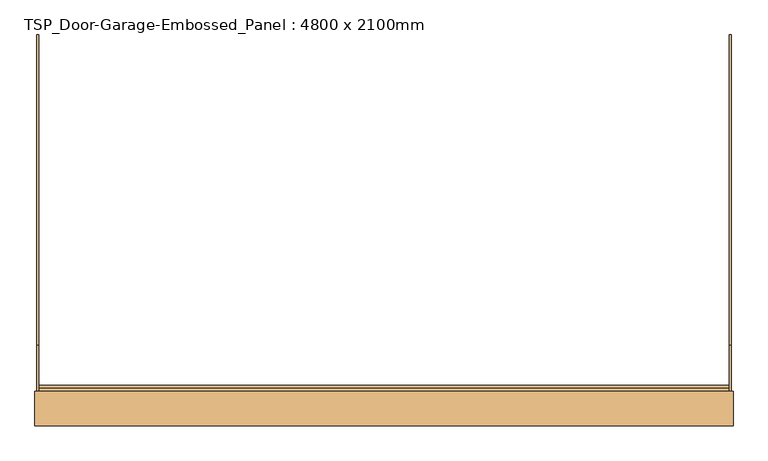
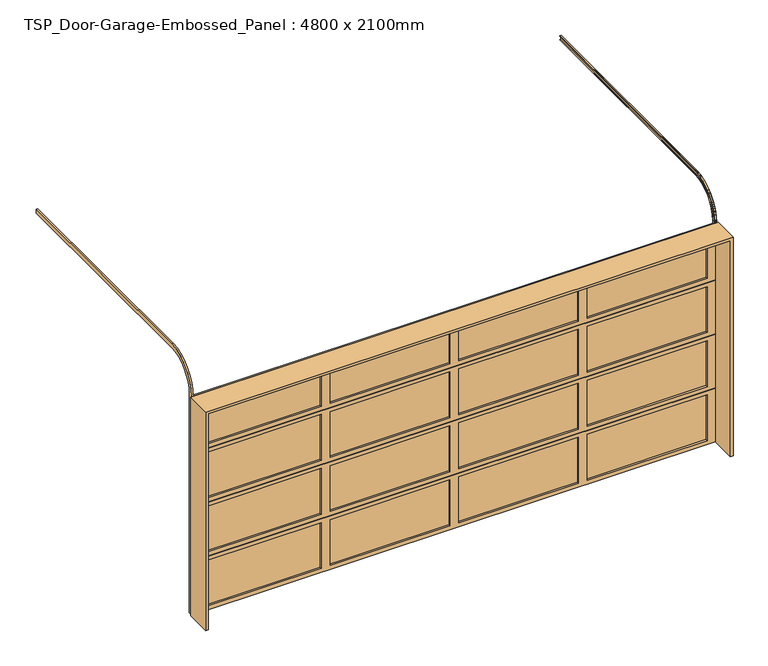
"""IFC4 building model written with IfcOpenShell, lengths in millimetres: door geometry, TSP_Door-Garage-Embossed_Panel : 4800 x 2100mm."""

from ifc_helpers import new_model, si_unit, frame, origin, place, context, project, spatial, polyline, circle_curve, outline, extrude, faceted_brep, source, transform, mapped, element, save
from ifc_brep_helpers import plane_surface, cylinder_surface, revolved_surface, advanced_brep


def tsp_door_garage_embossed_panel_4800_x_2100mm_f4924081(model_context):
    return source(origin(), model_context, "Body", "SolidModel", [
        extrude(outline(polyline([(1141.2666667, 140.0), (41.2666667, 140.0), (41.2666667, 146.35), (1141.2666667, 146.35), (1141.2666667, 140.0)])), frame((0.0, 0.0, 1615.0), z_axis=(0.0, 0.0, 1.0), x_axis=(1.0, 0.0, 0.0)), (0.0, 0.0, 1.0), 445.0),
        extrude(outline(polyline([(-41.2666667, 140.0), (-1141.2666667, 140.0), (-1141.2666667, 146.35), (-41.2666667, 146.35), (-41.2666667, 140.0)])), frame((0.0, 0.0, 1615.0), z_axis=(0.0, 0.0, 1.0), x_axis=(1.0, 0.0, 0.0)), (0.0, 0.0, 1.0), 445.0),
        extrude(outline(polyline([(2323.8, 140.0), (1223.8, 140.0), (1223.8, 146.35), (2323.8, 146.35), (2323.8, 140.0)])), frame((0.0, 0.0, 1615.0), z_axis=(0.0, 0.0, 1.0), x_axis=(1.0, 0.0, 0.0)), (0.0, 0.0, 1.0), 445.0),
        extrude(outline(polyline([(-1223.8, 140.0), (-2323.8, 140.0), (-2323.8, 146.35), (-1223.8, 146.35), (-1223.8, 140.0)])), frame((0.0, 0.0, 1615.0), z_axis=(0.0, 0.0, 1.0), x_axis=(1.0, 0.0, 0.0)), (0.0, 0.0, 1.0), 445.0),
        faceted_brep([(2400.0, 146.35, 2103.175), (2400.0, 146.35, 2096.825), (2400.0, 123.175, 2096.825), (2400.0, 123.175, 1575.0), (2400.0, 140.0, 1575.0), (2400.0, 140.0, 1581.35), (2400.0, 163.175, 1581.35), (2400.0, 163.175, 2103.175), (-2400.0, 163.175, 2103.175), (-2400.0, 163.175, 1581.35), (-2400.0, 140.0, 1581.35), (-2400.0, 140.0, 1575.0), (-2400.0, 123.175, 1575.0), (-2400.0, 123.175, 2096.825), (-2400.0, 146.35, 2096.825), (-2400.0, 146.35, 2103.175), (1223.8, 163.175, 2060.0), (1223.8, 163.175, 1615.0), (2323.8, 163.175, 1615.0), (2323.8, 163.175, 2060.0), (-1141.2666667, 163.175, 2060.0), (-1141.2666667, 163.175, 1615.0), (-41.2666667, 163.175, 1615.0), (-41.2666667, 163.175, 2060.0), (41.2666667, 163.175, 2060.0), (41.2666667, 163.175, 1615.0), (1141.2666667, 163.175, 1615.0), (1141.2666667, 163.175, 2060.0), (-2323.8, 163.175, 2060.0), (-2323.8, 163.175, 1615.0), (-1223.8, 163.175, 1615.0), (-1223.8, 163.175, 2060.0), (2323.8, 123.175, 2060.0), (2323.8, 123.175, 1615.0), (1223.8, 123.175, 1615.0), (1223.8, 123.175, 2060.0), (-41.2666667, 123.175, 2060.0), (-41.2666667, 123.175, 1615.0), (-1141.2666667, 123.175, 1615.0), (-1141.2666667, 123.175, 2060.0), (1141.2666667, 123.175, 2060.0), (1141.2666667, 123.175, 1615.0), (41.2666667, 123.175, 1615.0), (41.2666667, 123.175, 2060.0), (-1223.8, 123.175, 2060.0), (-1223.8, 123.175, 1615.0), (-2323.8, 123.175, 1615.0), (-2323.8, 123.175, 2060.0)], [[[0, 1, 2, 3, 4, 5, 6, 7]], [[8, 9, 10, 11, 12, 13, 14, 15]], [[7, 8, 15, 0]], [[6, 9, 8, 7], [16, 17, 18, 19], [20, 21, 22, 23], [24, 25, 26, 27], [28, 29, 30, 31]], [[5, 10, 9, 6]], [[4, 11, 10, 5]], [[3, 12, 11, 4]], [[2, 13, 12, 3], [32, 33, 34, 35], [36, 37, 38, 39], [40, 41, 42, 43], [44, 45, 46, 47]], [[1, 14, 13, 2]], [[0, 15, 14, 1]], [[16, 19, 32, 35]], [[35, 34, 17, 16]], [[34, 33, 18, 17]], [[19, 18, 33, 32]], [[20, 23, 36, 39]], [[39, 38, 21, 20]], [[38, 37, 22, 21]], [[23, 22, 37, 36]], [[24, 27, 40, 43]], [[43, 42, 25, 24]], [[42, 41, 26, 25]], [[27, 26, 41, 40]], [[28, 31, 44, 47]], [[47, 46, 29, 28]], [[46, 45, 30, 29]], [[31, 30, 45, 44]]]),
        extrude(outline(polyline([(1141.2666667, 140.0), (41.2666667, 140.0), (41.2666667, 146.35), (1141.2666667, 146.35), (1141.2666667, 140.0)])), frame((0.0, 0.0, 1090.0), z_axis=(0.0, 0.0, 1.0), x_axis=(1.0, 0.0, 0.0)), (0.0, 0.0, 1.0), 445.0),
        extrude(outline(polyline([(-41.2666667, 140.0), (-1141.2666667, 140.0), (-1141.2666667, 146.35), (-41.2666667, 146.35), (-41.2666667, 140.0)])), frame((0.0, 0.0, 1090.0), z_axis=(0.0, 0.0, 1.0), x_axis=(1.0, 0.0, 0.0)), (0.0, 0.0, 1.0), 445.0),
        extrude(outline(polyline([(2323.8, 140.0), (1223.8, 140.0), (1223.8, 146.35), (2323.8, 146.35), (2323.8, 140.0)])), frame((0.0, 0.0, 1090.0), z_axis=(0.0, 0.0, 1.0), x_axis=(1.0, 0.0, 0.0)), (0.0, 0.0, 1.0), 445.0),
        extrude(outline(polyline([(-1223.8, 140.0), (-2323.8, 140.0), (-2323.8, 146.35), (-1223.8, 146.35), (-1223.8, 140.0)])), frame((0.0, 0.0, 1090.0), z_axis=(0.0, 0.0, 1.0), x_axis=(1.0, 0.0, 0.0)), (0.0, 0.0, 1.0), 445.0),
        faceted_brep([(2400.0, 146.35, 1578.175), (2400.0, 146.35, 1571.825), (2400.0, 123.175, 1571.825), (2400.0, 123.175, 1050.0), (2400.0, 140.0, 1050.0), (2400.0, 140.0, 1056.35), (2400.0, 163.175, 1056.35), (2400.0, 163.175, 1578.175), (-2400.0, 163.175, 1578.175), (-2400.0, 163.175, 1056.35), (-2400.0, 140.0, 1056.35), (-2400.0, 140.0, 1050.0), (-2400.0, 123.175, 1050.0), (-2400.0, 123.175, 1571.825), (-2400.0, 146.35, 1571.825), (-2400.0, 146.35, 1578.175), (1223.8, 163.175, 1535.0), (1223.8, 163.175, 1090.0), (2323.8, 163.175, 1090.0), (2323.8, 163.175, 1535.0), (-1141.2666667, 163.175, 1535.0), (-1141.2666667, 163.175, 1090.0), (-41.2666667, 163.175, 1090.0), (-41.2666667, 163.175, 1535.0), (41.2666667, 163.175, 1535.0), (41.2666667, 163.175, 1090.0), (1141.2666667, 163.175, 1090.0), (1141.2666667, 163.175, 1535.0), (-2323.8, 163.175, 1535.0), (-2323.8, 163.175, 1090.0), (-1223.8, 163.175, 1090.0), (-1223.8, 163.175, 1535.0), (2323.8, 123.175, 1535.0), (2323.8, 123.175, 1090.0), (1223.8, 123.175, 1090.0), (1223.8, 123.175, 1535.0), (-41.2666667, 123.175, 1535.0), (-41.2666667, 123.175, 1090.0), (-1141.2666667, 123.175, 1090.0), (-1141.2666667, 123.175, 1535.0), (1141.2666667, 123.175, 1535.0), (1141.2666667, 123.175, 1090.0), (41.2666667, 123.175, 1090.0), (41.2666667, 123.175, 1535.0), (-1223.8, 123.175, 1535.0), (-1223.8, 123.175, 1090.0), (-2323.8, 123.175, 1090.0), (-2323.8, 123.175, 1535.0)], [[[0, 1, 2, 3, 4, 5, 6, 7]], [[8, 9, 10, 11, 12, 13, 14, 15]], [[7, 8, 15, 0]], [[6, 9, 8, 7], [16, 17, 18, 19], [20, 21, 22, 23], [24, 25, 26, 27], [28, 29, 30, 31]], [[5, 10, 9, 6]], [[4, 11, 10, 5]], [[3, 12, 11, 4]], [[2, 13, 12, 3], [32, 33, 34, 35], [36, 37, 38, 39], [40, 41, 42, 43], [44, 45, 46, 47]], [[1, 14, 13, 2]], [[0, 15, 14, 1]], [[16, 19, 32, 35]], [[35, 34, 17, 16]], [[34, 33, 18, 17]], [[19, 18, 33, 32]], [[20, 23, 36, 39]], [[39, 38, 21, 20]], [[38, 37, 22, 21]], [[23, 22, 37, 36]], [[24, 27, 40, 43]], [[43, 42, 25, 24]], [[42, 41, 26, 25]], [[27, 26, 41, 40]], [[28, 31, 44, 47]], [[47, 46, 29, 28]], [[46, 45, 30, 29]], [[31, 30, 45, 44]]]),
        extrude(outline(polyline([(1141.2666667, 140.0), (41.2666667, 140.0), (41.2666667, 146.35), (1141.2666667, 146.35), (1141.2666667, 140.0)])), frame((0.0, 0.0, 565.0), z_axis=(0.0, 0.0, 1.0), x_axis=(1.0, 0.0, 0.0)), (0.0, 0.0, 1.0), 445.0),
        extrude(outline(polyline([(-41.2666667, 140.0), (-1141.2666667, 140.0), (-1141.2666667, 146.35), (-41.2666667, 146.35), (-41.2666667, 140.0)])), frame((0.0, 0.0, 565.0), z_axis=(0.0, 0.0, 1.0), x_axis=(1.0, 0.0, 0.0)), (0.0, 0.0, 1.0), 445.0),
        extrude(outline(polyline([(2323.8, 140.0), (1223.8, 140.0), (1223.8, 146.35), (2323.8, 146.35), (2323.8, 140.0)])), frame((0.0, 0.0, 565.0), z_axis=(0.0, 0.0, 1.0), x_axis=(1.0, 0.0, 0.0)), (0.0, 0.0, 1.0), 445.0),
        extrude(outline(polyline([(-1223.8, 140.0), (-2323.8, 140.0), (-2323.8, 146.35), (-1223.8, 146.35), (-1223.8, 140.0)])), frame((0.0, 0.0, 565.0), z_axis=(0.0, 0.0, 1.0), x_axis=(1.0, 0.0, 0.0)), (0.0, 0.0, 1.0), 445.0),
        faceted_brep([(2400.0, 146.35, 1053.175), (2400.0, 146.35, 1046.825), (2400.0, 123.175, 1046.825), (2400.0, 123.175, 525.0), (2400.0, 140.0, 525.0), (2400.0, 140.0, 531.35), (2400.0, 163.175, 531.35), (2400.0, 163.175, 1053.175), (-2400.0, 163.175, 1053.175), (-2400.0, 163.175, 531.35), (-2400.0, 140.0, 531.35), (-2400.0, 140.0, 525.0), (-2400.0, 123.175, 525.0), (-2400.0, 123.175, 1046.825), (-2400.0, 146.35, 1046.825), (-2400.0, 146.35, 1053.175), (1223.8, 163.175, 1010.0), (1223.8, 163.175, 565.0), (2323.8, 163.175, 565.0), (2323.8, 163.175, 1010.0), (-1141.2666667, 163.175, 1010.0), (-1141.2666667, 163.175, 565.0), (-41.2666667, 163.175, 565.0), (-41.2666667, 163.175, 1010.0), (41.2666667, 163.175, 1010.0), (41.2666667, 163.175, 565.0), (1141.2666667, 163.175, 565.0), (1141.2666667, 163.175, 1010.0), (-2323.8, 163.175, 1010.0), (-2323.8, 163.175, 565.0), (-1223.8, 163.175, 565.0), (-1223.8, 163.175, 1010.0), (2323.8, 123.175, 1010.0), (2323.8, 123.175, 565.0), (1223.8, 123.175, 565.0), (1223.8, 123.175, 1010.0), (-41.2666667, 123.175, 1010.0), (-41.2666667, 123.175, 565.0), (-1141.2666667, 123.175, 565.0), (-1141.2666667, 123.175, 1010.0), (1141.2666667, 123.175, 1010.0), (1141.2666667, 123.175, 565.0), (41.2666667, 123.175, 565.0), (41.2666667, 123.175, 1010.0), (-1223.8, 123.175, 1010.0), (-1223.8, 123.175, 565.0), (-2323.8, 123.175, 565.0), (-2323.8, 123.175, 1010.0)], [[[0, 1, 2, 3, 4, 5, 6, 7]], [[8, 9, 10, 11, 12, 13, 14, 15]], [[7, 8, 15, 0]], [[6, 9, 8, 7], [16, 17, 18, 19], [20, 21, 22, 23], [24, 25, 26, 27], [28, 29, 30, 31]], [[5, 10, 9, 6]], [[4, 11, 10, 5]], [[3, 12, 11, 4]], [[2, 13, 12, 3], [32, 33, 34, 35], [36, 37, 38, 39], [40, 41, 42, 43], [44, 45, 46, 47]], [[1, 14, 13, 2]], [[0, 15, 14, 1]], [[16, 19, 32, 35]], [[35, 34, 17, 16]], [[34, 33, 18, 17]], [[19, 18, 33, 32]], [[20, 23, 36, 39]], [[39, 38, 21, 20]], [[38, 37, 22, 21]], [[23, 22, 37, 36]], [[24, 27, 40, 43]], [[43, 42, 25, 24]], [[42, 41, 26, 25]], [[27, 26, 41, 40]], [[28, 31, 44, 47]], [[47, 46, 29, 28]], [[46, 45, 30, 29]], [[31, 30, 45, 44]]]),
        extrude(outline(polyline([(1141.2666667, 140.0), (41.2666667, 140.0), (41.2666667, 146.35), (1141.2666667, 146.35), (1141.2666667, 140.0)])), frame((0.0, 0.0, 40.0), z_axis=(0.0, 0.0, 1.0), x_axis=(1.0, 0.0, 0.0)), (0.0, 0.0, 1.0), 445.0),
        extrude(outline(polyline([(-41.2666667, 140.0), (-1141.2666667, 140.0), (-1141.2666667, 146.35), (-41.2666667, 146.35), (-41.2666667, 140.0)])), frame((0.0, 0.0, 40.0), z_axis=(0.0, 0.0, 1.0), x_axis=(1.0, 0.0, 0.0)), (0.0, 0.0, 1.0), 445.0),
        extrude(outline(polyline([(2323.8, 140.0), (1223.8, 140.0), (1223.8, 146.35), (2323.8, 146.35), (2323.8, 140.0)])), frame((0.0, 0.0, 40.0), z_axis=(0.0, 0.0, 1.0), x_axis=(1.0, 0.0, 0.0)), (0.0, 0.0, 1.0), 445.0),
        extrude(outline(polyline([(-1223.8, 140.0), (-2323.8, 140.0), (-2323.8, 146.35), (-1223.8, 146.35), (-1223.8, 140.0)])), frame((0.0, 0.0, 40.0), z_axis=(0.0, 0.0, 1.0), x_axis=(1.0, 0.0, 0.0)), (0.0, 0.0, 1.0), 445.0),
        faceted_brep([(2400.0, 146.35, 528.175), (2400.0, 146.35, 521.825), (2400.0, 123.175, 521.825), (2400.0, 123.175, 0.0), (2400.0, 140.0, 0.0), (2400.0, 140.0, 6.35), (2400.0, 163.175, 6.35), (2400.0, 163.175, 528.175), (-2400.0, 163.175, 528.175), (-2400.0, 163.175, 6.35), (-2400.0, 140.0, 6.35), (-2400.0, 140.0, 0.0), (-2400.0, 123.175, 0.0), (-2400.0, 123.175, 521.825), (-2400.0, 146.35, 521.825), (-2400.0, 146.35, 528.175), (1223.8, 163.175, 485.0), (1223.8, 163.175, 40.0), (2323.8, 163.175, 40.0), (2323.8, 163.175, 485.0), (-1141.2666667, 163.175, 485.0), (-1141.2666667, 163.175, 40.0), (-41.2666667, 163.175, 40.0), (-41.2666667, 163.175, 485.0), (41.2666667, 163.175, 485.0), (41.2666667, 163.175, 40.0), (1141.2666667, 163.175, 40.0), (1141.2666667, 163.175, 485.0), (-2323.8, 163.175, 485.0), (-2323.8, 163.175, 40.0), (-1223.8, 163.175, 40.0), (-1223.8, 163.175, 485.0), (2323.8, 123.175, 485.0), (2323.8, 123.175, 40.0), (1223.8, 123.175, 40.0), (1223.8, 123.175, 485.0), (-41.2666667, 123.175, 485.0), (-41.2666667, 123.175, 40.0), (-1141.2666667, 123.175, 40.0), (-1141.2666667, 123.175, 485.0), (1141.2666667, 123.175, 485.0), (1141.2666667, 123.175, 40.0), (41.2666667, 123.175, 40.0), (41.2666667, 123.175, 485.0), (-1223.8, 123.175, 485.0), (-1223.8, 123.175, 40.0), (-2323.8, 123.175, 40.0), (-2323.8, 123.175, 485.0)], [[[0, 1, 2, 3, 4, 5, 6, 7]], [[8, 9, 10, 11, 12, 13, 14, 15]], [[7, 8, 15, 0]], [[6, 9, 8, 7], [16, 17, 18, 19], [20, 21, 22, 23], [24, 25, 26, 27], [28, 29, 30, 31]], [[5, 10, 9, 6]], [[4, 11, 10, 5]], [[3, 12, 11, 4]], [[2, 13, 12, 3], [32, 33, 34, 35], [36, 37, 38, 39], [40, 41, 42, 43], [44, 45, 46, 47]], [[1, 14, 13, 2]], [[0, 15, 14, 1]], [[16, 19, 32, 35]], [[35, 34, 17, 16]], [[34, 33, 18, 17]], [[19, 18, 33, 32]], [[20, 23, 36, 39]], [[39, 38, 21, 20]], [[38, 37, 22, 21]], [[23, 22, 37, 36]], [[24, 27, 40, 43]], [[43, 42, 25, 24]], [[42, 41, 26, 25]], [[27, 26, 41, 40]], [[28, 31, 44, 47]], [[47, 46, 29, 28]], [[46, 45, 30, 29]], [[31, 30, 45, 44]]]),
        extrude(outline(polyline([(0.0, 2425.0), (2125.0, 2425.0), (2125.0, -2425.0), (0.0, -2425.0), (0.0, -2400.0), (2100.0, -2400.0), (2100.0, 2400.0), (0.0, 2400.0), (0.0, 2425.0)])), frame((0.0, -116.825, 0.0), z_axis=(0.0, 1.0, 0.0), x_axis=(0.0, 0.0, 1.0)), (0.0, 0.0, 1.0), 240.0),
        advanced_brep(
        [(2412.7, 163.175, 0.0), (2412.7, 123.175, 0.0), (2400.0, 123.175, 0.0), (2400.0, 126.375, 0.0), (2409.525, 126.375, 0.0), (2409.525, 160.0, 0.0), (2400.0, 160.0, 0.0), (2400.0, 163.175, 0.0), (2400.0, 163.175, 2125.0), (2412.7, 163.175, 2125.0), (2400.0, 160.0, 2125.0), (2400.0, 442.575, 2407.575), (2400.0, 2601.575, 2407.575), (2400.0, 2601.575, 2404.4), (2400.0, 442.575, 2404.4), (2409.525, 160.0, 2125.0), (2409.525, 126.375, 2125.0), (2409.525, 442.575, 2441.2), (2409.525, 2601.575, 2441.2), (2409.525, 2601.575, 2407.575), (2409.525, 442.575, 2407.575), (2400.0, 126.375, 2125.0), (2400.0, 123.175, 2125.0), (2400.0, 442.575, 2444.4), (2400.0, 2601.575, 2444.4), (2400.0, 2601.575, 2441.2), (2400.0, 442.575, 2441.2), (2412.7, 123.175, 2125.0), (2412.7, 442.575, 2404.4), (2412.7, 2601.575, 2404.4), (2412.7, 2601.575, 2444.4), (2412.7, 442.575, 2444.4)],
        [
            (0, 1),
            (1, 2),
            (2, 3),
            (3, 4),
            (4, 5),
            (5, 6),
            (6, 7),
            (7, 0),
            (7, 8),
            (8, 9),
            (9, 0),
            (6, 10),
            (10, 11, circle_curve(frame((2400.0, 442.575, 2125.0), z_axis=(-1.0, 0.0, 0.0), x_axis=(0.0, -1.0, 0.0)), 282.575)),
            (11, 12),
            (12, 13),
            (13, 14),
            (14, 8, circle_curve(frame((2400.0, 442.575, 2125.0), z_axis=(1.0, 0.0, 0.0), x_axis=(0.0, -1.0, 0.0)), 279.4)),
            (5, 15),
            (15, 10),
            (4, 16),
            (16, 17, circle_curve(frame((2409.525, 442.575, 2125.0), z_axis=(-1.0, 0.0, 0.0), x_axis=(0.0, -1.0, 0.0)), 316.2)),
            (17, 18),
            (18, 19),
            (19, 20),
            (20, 15, circle_curve(frame((2409.525, 442.575, 2125.0), z_axis=(1.0, 0.0, 0.0), x_axis=(0.0, -1.0, 0.0)), 282.575)),
            (3, 21),
            (21, 16),
            (2, 22),
            (22, 23, circle_curve(frame((2400.0, 442.575, 2125.0), z_axis=(-1.0, 0.0, 0.0), x_axis=(0.0, -1.0, 0.0)), 319.4)),
            (23, 24),
            (24, 25),
            (25, 26),
            (26, 21, circle_curve(frame((2400.0, 442.575, 2125.0), z_axis=(1.0, 0.0, 0.0), x_axis=(0.0, -1.0, 0.0)), 316.2)),
            (1, 27),
            (27, 22),
            (9, 28, circle_curve(frame((2412.7, 442.575, 2125.0), z_axis=(-1.0, 0.0, 0.0), x_axis=(0.0, -1.0, 0.0)), 279.4)),
            (28, 29),
            (29, 30),
            (30, 31),
            (31, 27, circle_curve(frame((2412.7, 442.575, 2125.0), z_axis=(1.0, 0.0, 0.0), x_axis=(0.0, -1.0, 0.0)), 319.4)),
            (14, 28),
            (20, 11),
            (26, 17),
            (31, 23),
            (29, 13),
            (12, 19),
            (18, 25),
            (24, 30),
        ],
        [
            plane_surface(frame((0.0, 163.175, 0.0), z_axis=(0.0, 0.0, -1.0), x_axis=(1.0, 0.0, 0.0))),
            plane_surface(frame((2412.7, 163.175, 0.0), z_axis=(0.0, 1.0, 0.0), x_axis=(0.0, 0.0, 1.0))),
            plane_surface(frame((2400.0, 163.175, 0.0), z_axis=(-1.0, 0.0, 0.0), x_axis=(0.0, 0.0, 1.0))),
            plane_surface(frame((2400.0, 160.0, 0.0), z_axis=(0.0, -1.0, 0.0), x_axis=(0.0, 0.0, 1.0))),
            plane_surface(frame((2409.525, 160.0, 0.0), z_axis=(-1.0, 0.0, 0.0), x_axis=(0.0, 0.0, 1.0))),
            plane_surface(frame((2409.525, 126.375, 0.0), z_axis=(0.0, 1.0, 0.0), x_axis=(0.0, 0.0, 1.0))),
            plane_surface(frame((2400.0, 126.375, 0.0), z_axis=(-1.0, 0.0, 0.0), x_axis=(0.0, 0.0, 1.0))),
            plane_surface(frame((2400.0, 123.175, 0.0), z_axis=(0.0, -1.0, 0.0), x_axis=(0.0, 0.0, 1.0))),
            plane_surface(frame((2412.7, 123.175, 0.0), z_axis=(1.0, 0.0, 0.0), x_axis=(0.0, 0.0, 1.0))),
            revolved_surface(polyline([(2412.7, 163.175, 2125.0), (2400.0, 163.175, 2125.0)]), (0.0, 442.575, 2125.0), (1.0, 0.0, 0.0)),
            cylinder_surface(frame((0.0, 442.575, 2125.0), z_axis=(1.0, 0.0, 0.0), x_axis=(0.0, -1.0, 0.0)), 282.575),
            revolved_surface(polyline([(2409.525, 126.375, 2125.0), (2400.0, 126.375, 2125.0)]), (0.0, 442.575, 2125.0), (1.0, 0.0, 0.0)),
            cylinder_surface(frame((0.0, 442.575, 2125.0), z_axis=(1.0, 0.0, 0.0), x_axis=(0.0, -1.0, 0.0)), 319.4),
            plane_surface(frame((0.0, 2601.575, 2404.4), z_axis=(0.0, 1.0, 0.0), x_axis=(1.0, 0.0, 0.0))),
            plane_surface(frame((2412.7, 442.575, 2404.4), z_axis=(0.0, 0.0, -1.0), x_axis=(0.0, 1.0, 0.0))),
            plane_surface(frame((2400.0, 442.575, 2407.575), z_axis=(0.0, 0.0, 1.0), x_axis=(0.0, 1.0, 0.0))),
            plane_surface(frame((2409.525, 442.575, 2441.2), z_axis=(0.0, 0.0, -1.0), x_axis=(0.0, 1.0, 0.0))),
            plane_surface(frame((2400.0, 442.575, 2444.4), z_axis=(0.0, 0.0, 1.0), x_axis=(0.0, 1.0, 0.0))),
        ],
        [
            (0, [[1, 2, 3, 4, 5, 6, 7, 8]]),
            (1, [[9, 10, 11, -8]]),
            (2, [[12, 13, 14, 15, 16, 17, -9, -7]]),
            (3, [[18, 19, -12, -6]]),
            (4, [[20, 21, 22, 23, 24, 25, -18, -5]]),
            (5, [[26, 27, -20, -4]]),
            (6, [[28, 29, 30, 31, 32, 33, -26, -3]]),
            (7, [[34, 35, -28, -2]]),
            (8, [[-11, 36, 37, 38, 39, 40, -34, -1]]),
            (9, [[41, -36, -10, -17]]),
            (10, [[42, -13, -19, -25]]),
            (11, [[43, -21, -27, -33]]),
            (12, [[44, -29, -35, -40]]),
            (13, [[45, -15, 46, -23, 47, -31, 48, -38]]),
            (14, [[-16, -45, -37, -41]]),
            (15, [[-24, -46, -14, -42]]),
            (16, [[-32, -47, -22, -43]]),
            (17, [[-39, -48, -30, -44]]),
        ],
    ),
        advanced_brep(
        [(-2412.7, 163.175, 0.0), (-2400.0, 163.175, 0.0), (-2400.0, 160.0, 0.0), (-2409.525, 160.0, 0.0), (-2409.525, 126.375, 0.0), (-2400.0, 126.375, 0.0), (-2400.0, 123.175, 0.0), (-2412.7, 123.175, 0.0), (-2412.7, 123.175, 2125.0), (-2412.7, 442.575, 2444.4), (-2412.7, 2601.575, 2444.4), (-2412.7, 2601.575, 2404.4), (-2412.7, 442.575, 2404.4), (-2412.7, 163.175, 2125.0), (-2400.0, 123.175, 2125.0), (-2400.0, 126.375, 2125.0), (-2400.0, 442.575, 2441.2), (-2400.0, 2601.575, 2441.2), (-2400.0, 2601.575, 2444.4), (-2400.0, 442.575, 2444.4), (-2409.525, 126.375, 2125.0), (-2409.525, 160.0, 2125.0), (-2409.525, 442.575, 2407.575), (-2409.525, 2601.575, 2407.575), (-2409.525, 2601.575, 2441.2), (-2409.525, 442.575, 2441.2), (-2400.0, 160.0, 2125.0), (-2400.0, 163.175, 2125.0), (-2400.0, 442.575, 2404.4), (-2400.0, 2601.575, 2404.4), (-2400.0, 2601.575, 2407.575), (-2400.0, 442.575, 2407.575)],
        [
            (0, 1),
            (1, 2),
            (2, 3),
            (3, 4),
            (4, 5),
            (5, 6),
            (6, 7),
            (7, 0),
            (7, 8),
            (8, 9, circle_curve(frame((-2412.7, 442.575, 2125.0), z_axis=(-1.0, 0.0, 0.0), x_axis=(0.0, -1.0, 0.0)), 319.4)),
            (9, 10),
            (10, 11),
            (11, 12),
            (12, 13, circle_curve(frame((-2412.7, 442.575, 2125.0), z_axis=(1.0, 0.0, 0.0), x_axis=(0.0, -1.0, 0.0)), 279.4)),
            (13, 0),
            (6, 14),
            (14, 8),
            (5, 15),
            (15, 16, circle_curve(frame((-2400.0, 442.575, 2125.0), z_axis=(-1.0, 0.0, 0.0), x_axis=(0.0, -1.0, 0.0)), 316.2)),
            (16, 17),
            (17, 18),
            (18, 19),
            (19, 14, circle_curve(frame((-2400.0, 442.575, 2125.0), z_axis=(1.0, 0.0, 0.0), x_axis=(0.0, -1.0, 0.0)), 319.4)),
            (4, 20),
            (20, 15),
            (3, 21),
            (21, 22, circle_curve(frame((-2409.525, 442.575, 2125.0), z_axis=(-1.0, 0.0, 0.0), x_axis=(0.0, -1.0, 0.0)), 282.575)),
            (22, 23),
            (23, 24),
            (24, 25),
            (25, 20, circle_curve(frame((-2409.525, 442.575, 2125.0), z_axis=(1.0, 0.0, 0.0), x_axis=(0.0, -1.0, 0.0)), 316.2)),
            (2, 26),
            (26, 21),
            (1, 27),
            (27, 28, circle_curve(frame((-2400.0, 442.575, 2125.0), z_axis=(-1.0, 0.0, 0.0), x_axis=(0.0, -1.0, 0.0)), 279.4)),
            (28, 29),
            (29, 30),
            (30, 31),
            (31, 26, circle_curve(frame((-2400.0, 442.575, 2125.0), z_axis=(1.0, 0.0, 0.0), x_axis=(0.0, -1.0, 0.0)), 282.575)),
            (13, 27),
            (19, 9),
            (25, 16),
            (31, 22),
            (12, 28),
            (10, 18),
            (17, 24),
            (23, 30),
            (29, 11),
        ],
        [
            plane_surface(frame((0.0, 163.175, 0.0), z_axis=(0.0, 0.0, -1.0), x_axis=(1.0, 0.0, 0.0))),
            plane_surface(frame((-2412.7, 163.175, 0.0), z_axis=(-1.0, 0.0, 0.0), x_axis=(0.0, 0.0, 1.0))),
            plane_surface(frame((-2412.7, 123.175, 0.0), z_axis=(0.0, -1.0, 0.0), x_axis=(0.0, 0.0, 1.0))),
            plane_surface(frame((-2400.0, 123.175, 0.0), z_axis=(1.0, 0.0, 0.0), x_axis=(0.0, 0.0, 1.0))),
            plane_surface(frame((-2400.0, 126.375, 0.0), z_axis=(0.0, 1.0, 0.0), x_axis=(0.0, 0.0, 1.0))),
            plane_surface(frame((-2409.525, 126.375, 0.0), z_axis=(1.0, 0.0, 0.0), x_axis=(0.0, 0.0, 1.0))),
            plane_surface(frame((-2409.525, 160.0, 0.0), z_axis=(0.0, -1.0, 0.0), x_axis=(0.0, 0.0, 1.0))),
            plane_surface(frame((-2400.0, 160.0, 0.0), z_axis=(1.0, 0.0, 0.0), x_axis=(0.0, 0.0, 1.0))),
            plane_surface(frame((-2400.0, 163.175, 0.0), z_axis=(0.0, 1.0, 0.0), x_axis=(0.0, 0.0, 1.0))),
            cylinder_surface(frame((0.0, 442.575, 2125.0), z_axis=(1.0, 0.0, 0.0), x_axis=(0.0, -1.0, 0.0)), 319.4),
            revolved_surface(polyline([(-2400.0, 126.375, 2125.0), (-2409.525, 126.375, 2125.0)]), (0.0, 442.575, 2125.0), (1.0, 0.0, 0.0)),
            cylinder_surface(frame((0.0, 442.575, 2125.0), z_axis=(1.0, 0.0, 0.0), x_axis=(0.0, -1.0, 0.0)), 282.575),
            revolved_surface(polyline([(-2400.0, 163.175, 2125.0), (-2412.7, 163.175, 2125.0)]), (0.0, 442.575, 2125.0), (1.0, 0.0, 0.0)),
            plane_surface(frame((0.0, 2601.575, 2404.4), z_axis=(0.0, 1.0, 0.0), x_axis=(1.0, 0.0, 0.0))),
            plane_surface(frame((-2412.7, 442.575, 2444.4), z_axis=(0.0, 0.0, 1.0), x_axis=(0.0, 1.0, 0.0))),
            plane_surface(frame((-2400.0, 442.575, 2441.2), z_axis=(0.0, 0.0, -1.0), x_axis=(0.0, 1.0, 0.0))),
            plane_surface(frame((-2409.525, 442.575, 2407.575), z_axis=(0.0, 0.0, 1.0), x_axis=(0.0, 1.0, 0.0))),
            plane_surface(frame((-2400.0, 442.575, 2404.4), z_axis=(0.0, 0.0, -1.0), x_axis=(0.0, 1.0, 0.0))),
        ],
        [
            (0, [[1, 2, 3, 4, 5, 6, 7, 8]]),
            (1, [[9, 10, 11, 12, 13, 14, 15, -8]]),
            (2, [[16, 17, -9, -7]]),
            (3, [[18, 19, 20, 21, 22, 23, -16, -6]]),
            (4, [[24, 25, -18, -5]]),
            (5, [[26, 27, 28, 29, 30, 31, -24, -4]]),
            (6, [[32, 33, -26, -3]]),
            (7, [[34, 35, 36, 37, 38, 39, -32, -2]]),
            (8, [[-15, 40, -34, -1]]),
            (9, [[41, -10, -17, -23]]),
            (10, [[42, -19, -25, -31]]),
            (11, [[43, -27, -33, -39]]),
            (12, [[44, -35, -40, -14]]),
            (13, [[-12, 45, -21, 46, -29, 47, -37, 48]]),
            (14, [[-22, -45, -11, -41]]),
            (15, [[-30, -46, -20, -42]]),
            (16, [[-38, -47, -28, -43]]),
            (17, [[-13, -48, -36, -44]]),
        ],
    ),
    ])


if __name__ == "__main__":
    model = new_model("IFC4")
    model_context = context("Model", 3, world=origin())
    ifc_project = project(units=[si_unit("LENGTHUNIT", "METRE", prefix="MILLI")], contexts=[model_context])
    site = spatial("IfcSite", under=ifc_project)
    building = spatial("IfcBuilding", under=site)
    placement = place(None, origin())
    tsp_door_garage_embossed_panel_4800_x_2100mm_shape = tsp_door_garage_embossed_panel_4800_x_2100mm_f4924081(model_context)
    element("IfcDoor", 1, ObjectType="TSP_Door-Garage-Embossed_Panel : 4800 x 2100mm", at=placement, inside=building, context=model_context, shape_type="MappedRepresentation", body=[
        mapped(tsp_door_garage_embossed_panel_4800_x_2100mm_shape, transform((0.0, 0.0, 0.0), x_axis=(1.0, 0.0, 0.0), y_axis=(0.0, 1.0, 0.0), z_axis=(0.0, 0.0, 1.0))),
    ])
    save(model, "model.ifc")

# Revit data of these elements
# Type "TSP_Door-Garage-Embossed_Panel : 4800 x 2100mm"
#   Model = "TSP_DOOR01AG"
#   Type Mark = "62"
#   Analytic Construction = "Wooden"
#   Thickness = 40 mm
#   Thermal Resistance (R) = 0.455703 (m²·K)/W
#   Rough Width = 4850 mm
#   Rough Height = 2125 mm
#   Panel Height = 525 mm
#   Height = 2100 mm
#   Width = 4800 mm
#   Heat Transfer Coefficient (U) = 2.19465 W/(m²·K)
#   Panels = 4
#   Function = 1
#   Exterior Trim [instance default] = yes
#   Trim Material = Cherry
#   Panel Material = Cherry
#   Frame Material = Cherry
#   Visual Light Transmittance = 0
#   Solar Heat Gain Coefficient = 0
#   Wall Closure = (empty or 0)
#   Assembly Code = ""
# Element 1 (IfcDoor, "TSP_Door-Garage-Embossed_Panel : 4800 x 2100mm")
#   Materials on its faces: "Cherry"
# Materials
#   "Cherry": class "Wood", colour RGB 226 177 128, transparency 0, Description = "Prunus Serotina", Cost = 0
